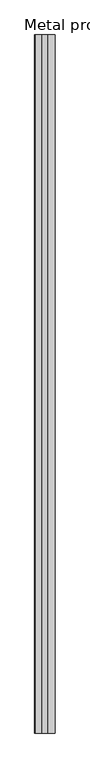
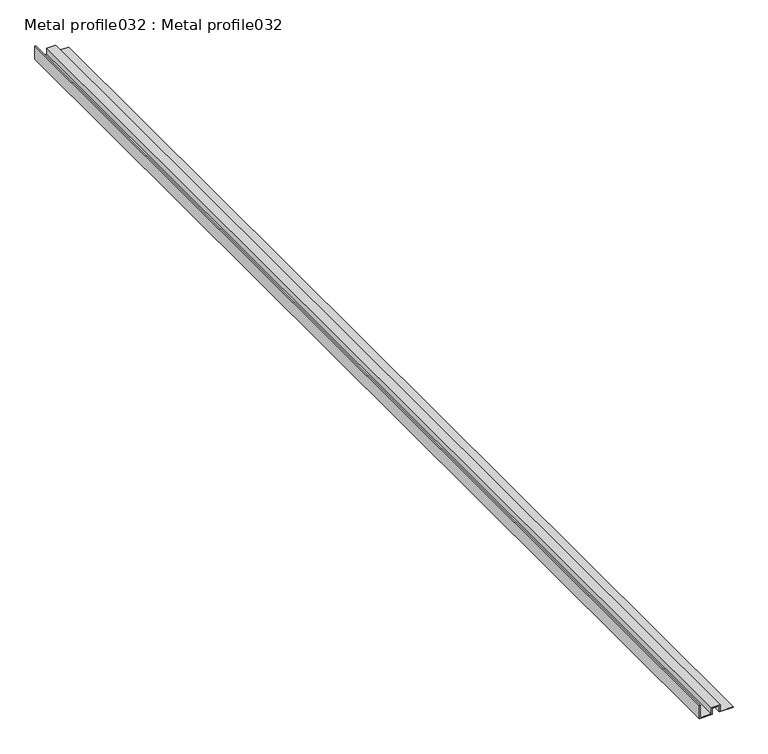
"""IFC4 building model written with IfcOpenShell, lengths in millimetres: proxy geometry, Metal profile032 : Metal profile032."""

from ifc_helpers import new_model, si_unit, frame, origin, place, context, project, spatial, polyline, outline, extrude, source, transform, mapped, element, save


def metal_profile032_metal_profile032_b3f8fbd6(model_context):
    return source(origin(), model_context, "Body", "SweptSolid", [
        extrude(outline(polyline([(39542.6175708, -9915.4255764), (39542.6175708, -9893.2005764), (39554.0475708, -9893.2005764), (39554.0475708, -9880.5005764), (39542.6175708, -9880.5005764), (39542.6175708, -9856.7873925), (39543.8975708, -9856.7873925), (39543.8975708, -9879.2205764), (39555.3275708, -9879.2205764), (39555.3275708, -9894.4805764), (39543.8975708, -9894.4805764), (39543.8975708, -9914.1455764), (39566.4183323, -9914.1455764), (39566.4183323, -9915.4255764), (39542.6175708, -9915.4255764)])), frame((0.0, 7982.1531721, 0.0), z_axis=(0.0, 1.0, 0.0), x_axis=(0.0, 0.0, 1.0)), (0.0, 0.0, 1.0), 2000.0),
    ])


if __name__ == "__main__":
    model = new_model("IFC4")
    model_context = context("Model", 3, world=origin())
    ifc_project = project(units=[si_unit("LENGTHUNIT", "METRE", prefix="MILLI")], contexts=[model_context])
    site = spatial("IfcSite", under=ifc_project)
    building = spatial("IfcBuilding", under=site)
    placement = place(None, origin())
    metal_profile032_metal_profile032_shape = metal_profile032_metal_profile032_b3f8fbd6(model_context)
    element("IfcBuildingElementProxy", 1, Name="Metal profile032 : Metal profile032", ObjectType="Metal profile032 : Metal profile032", at=placement, inside=building, context=model_context, shape_type="MappedRepresentation", body=[
        mapped(metal_profile032_metal_profile032_shape, transform((0.0, 0.0, 0.0), x_axis=(1.0, 0.0, 0.0), y_axis=(0.0, 1.0, 0.0), z_axis=(0.0, 0.0, 1.0))),
    ])
    save(model, "model.ifc")

# Revit data of these elements
# Type "Metal profile032 : Metal profile032"
#   NameOverride = "Metal profile032"
# Element 1 (IfcBuildingElementProxy, "Metal profile032 : Metal profile032")
#   Materials on its faces: "16 GA. COPPER SOFFIT DRIP SCREED"
# Materials
#   "16 GA. COPPER SOFFIT DRIP SCREED": class "Unassigned", colour RGB 255 217 0, transparency 0
